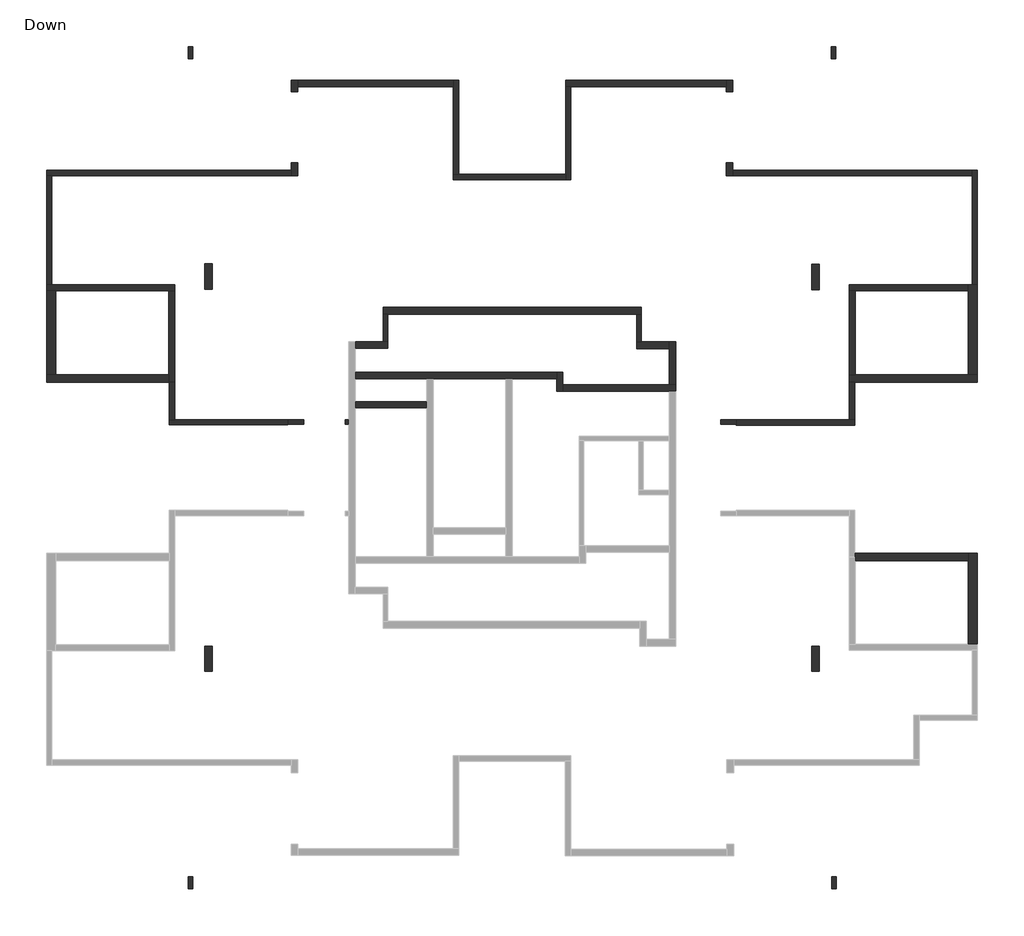
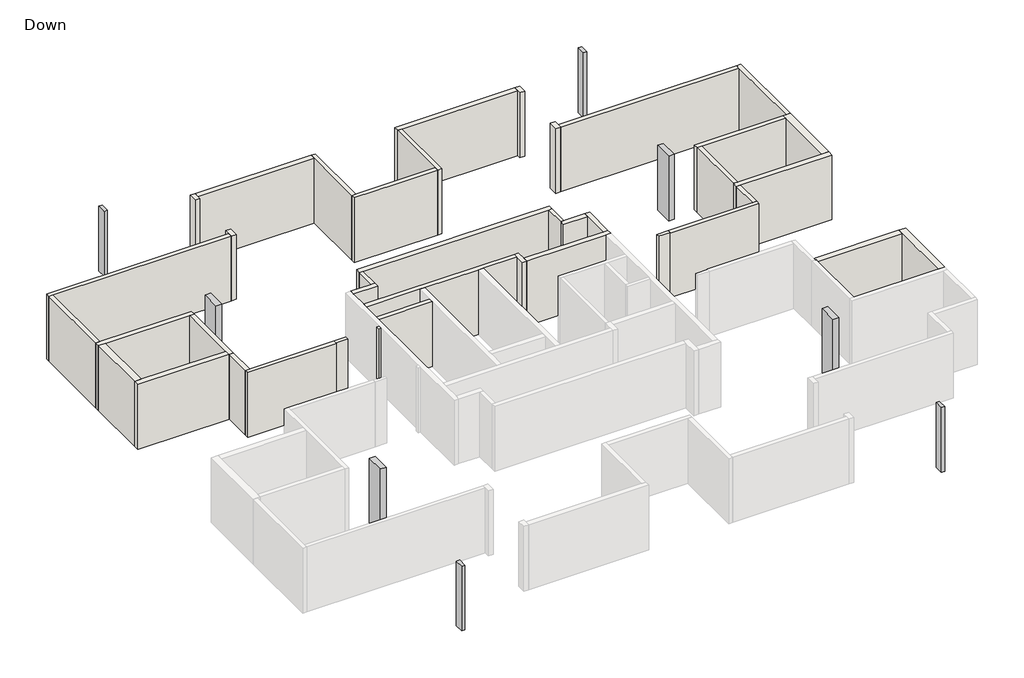
# One storey, part 2 of 2: 40 walls, 8 columns.
"""IFC4 building model written with IfcOpenShell, lengths in millimetres."""

from ifc_helpers import new_model, si_unit, origin, place, context, project, spatial, faceted_brep, element, save

model = new_model("IFC4")

# Units and contexts
model_context = context("Model", 3, world=origin())
ifc_project = project(units=[si_unit("LENGTHUNIT", "METRE", prefix="MILLI")], contexts=[model_context])

# Site, building, storey
site = spatial("IfcSite", under=ifc_project)
building = spatial("IfcBuilding", under=site)
storey = spatial("IfcBuildingStorey", under=building, Name="Down", Elevation=0.0)

# Columns
placement = place(None, origin())
element("IfcColumn", 1, ObjectType="Concrete Rectengular Column : 15/40", at=placement, inside=storey, context=model_context, shape_type="Brep", body=[
    faceted_brep([(7161.4479352, -14720.0113915, 0.0), (7161.4479352, -15120.0113915, 0.0), (7011.4479352, -15120.0113915, 0.0), (7011.4479352, -14720.0113915, 0.0), (7161.4479352, -14720.0113915, 3070.0), (7161.4479352, -15120.0113915, 3070.0), (7161.4479352, -14720.0113915, 2870.0), (7011.4479352, -15120.0113915, 3070.0), (7011.4479352, -15120.0113915, 2870.0), (7011.4479352, -14720.0113915, 3070.0), (7011.4479352, -14720.0113915, 2870.0)], [[[0, 1, 2, 3]], [[4, 5, 1, 0, 6]], [[5, 7, 8, 2, 1]], [[7, 9, 10, 3, 2, 8]], [[9, 4, 6, 0, 3, 10]], [[4, 9, 7, 5]]]),
])
element("IfcColumn", 2, ObjectType="Concrete Rectengular Column : 15/40", at=placement, inside=storey, context=model_context, shape_type="Brep", body=[
    faceted_brep([(-14313.9862657, -14720.0113915, 0.0), (-14313.9862657, -15120.0113915, 0.0), (-14463.9862657, -15120.0113915, 0.0), (-14463.9862657, -14720.0113915, 0.0), (-14313.9862657, -14720.0113915, 3070.0), (-14313.9862657, -15120.0113915, 3070.0), (-14313.9862657, -15120.0113915, 2870.0), (-14313.9862657, -14720.0113915, 2870.0), (-14463.9862657, -15120.0113915, 3070.0), (-14463.9862657, -14720.0113915, 3070.0), (-14463.9862657, -14720.0113915, 2870.0)], [[[0, 1, 2, 3]], [[4, 5, 6, 1, 0, 7]], [[5, 8, 2, 1, 6]], [[8, 9, 10, 3, 2]], [[9, 4, 7, 0, 3, 10]], [[4, 9, 8, 5]]]),
])
element("IfcColumn", 3, ObjectType="Concrete Rectengular Column : 15/40", at=placement, inside=storey, context=model_context, shape_type="Brep", body=[
    faceted_brep([(-14317.8223989, 12998.5060921, 0.0), (-14317.8223989, 12598.5060921, 0.0), (-14467.8223989, 12598.5060921, 0.0), (-14467.8223989, 12998.5060921, 0.0), (-14317.8223989, 12998.5060921, 3070.0), (-14317.8223989, 12598.5060921, 3070.0), (-14317.8223989, 12598.5060921, 2870.0), (-14467.8223989, 12598.5060921, 3070.0), (-14467.8223989, 12598.5060921, 2870.0), (-14467.8223989, 12998.5060921, 3070.0)], [[[0, 1, 2, 3]], [[4, 5, 6, 1, 0]], [[5, 7, 8, 2, 1, 6]], [[7, 9, 3, 2, 8]], [[9, 4, 0, 3]], [[4, 9, 7, 5]]]),
])
element("IfcColumn", 4, ObjectType="Concrete Rectengular Column : 15/40", at=placement, inside=storey, context=model_context, shape_type="Brep", body=[
    faceted_brep([(7142.0982792, 12598.507588, 0.0), (6992.0982792, 12598.507588, 0.0), (6992.0982792, 12998.507588, 0.0), (7142.0982792, 12998.507588, 0.0), (7142.0982792, 12598.507588, 3070.0), (7142.0982792, 12598.507588, 2870.0), (7142.0982792, 12998.507588, 3070.0), (6992.0982792, 12998.507588, 2870.0), (6992.0982792, 12998.507588, 3070.0), (6992.0982792, 12598.507588, 2870.0), (6992.0982792, 12598.507588, 3070.0)], [[[0, 1, 2, 3]], [[4, 5, 0, 3, 6]], [[6, 3, 2, 7, 8]], [[8, 7, 2, 1, 9, 10]], [[10, 9, 1, 0, 5, 4]], [[4, 6, 8, 10]]]),
])
element("IfcColumn", 5, ObjectType="Concrete Rectengular Column : 25/85", at=placement, inside=storey, context=model_context, shape_type="Brep", body=[
    faceted_brep([(-13656.3416868, -7010.4989795, 0.0), (-13656.3416868, -7860.4989795, 0.0), (-13906.3416868, -7860.4989795, 0.0), (-13906.3416868, -7010.4989795, 0.0), (-13656.3416868, -7010.4989795, 3070.0), (-13656.3416868, -7860.4989795, 3070.0), (-13656.3416868, -7860.4989795, 2870.0), (-13656.3416868, -7010.4989795, 2870.0), (-13906.3416868, -7860.4989795, 3070.0), (-13906.3416868, -7860.4989795, 2870.0), (-13906.3416868, -7010.4989795, 3070.0), (-13906.3416868, -7010.4989795, 2870.0)], [[[0, 1, 2, 3]], [[4, 5, 6, 1, 0, 7]], [[5, 8, 9, 2, 1, 6]], [[8, 10, 11, 3, 2, 9]], [[10, 4, 7, 0, 3, 11]], [[4, 10, 8, 5]]]),
])
element("IfcColumn", 6, ObjectType="Concrete Rectengular Column : 25/85", at=placement, inside=storey, context=model_context, shape_type="Brep", body=[
    faceted_brep([(6603.8022343, -7010.4989795, 0.0), (6603.8022343, -7860.4989795, 0.0), (6353.8022343, -7860.4989795, 0.0), (6353.8022343, -7010.4989795, 0.0), (6603.8022343, -7010.4989795, 3070.0), (6603.8022343, -7860.4989795, 3070.0), (6603.8022343, -7860.4989795, 2870.0), (6603.8022343, -7010.4989795, 2870.0), (6353.8022343, -7860.4989795, 3070.0), (6353.8022343, -7860.4989795, 2870.0), (6353.8022343, -7010.4989795, 3070.0), (6353.8022343, -7010.4989795, 2870.0)], [[[0, 1, 2, 3]], [[4, 5, 6, 1, 0, 7]], [[5, 8, 9, 2, 1, 6]], [[8, 10, 11, 3, 2, 9]], [[10, 4, 7, 0, 3, 11]], [[4, 10, 8, 5]]]),
])
element("IfcColumn", 7, ObjectType="Concrete Rectengular Column : 25/85", at=placement, inside=storey, context=model_context, shape_type="Brep", body=[
    faceted_brep([(-13656.3416868, 5740.9327236, 0.0), (-13656.3416868, 4890.9327236, 0.0), (-13906.3416868, 4890.9327236, 0.0), (-13906.3416868, 5740.9327236, 0.0), (-13656.3416868, 5740.9327236, 3070.0), (-13656.3416868, 4890.9327236, 3070.0), (-13656.3416868, 4890.9327236, 2870.0), (-13656.3416868, 5740.9327236, 2870.0), (-13906.3416868, 4890.9327236, 3070.0), (-13906.3416868, 4890.9327236, 2870.0), (-13906.3416868, 5740.9327236, 3070.0), (-13906.3416868, 5740.9327236, 2870.0)], [[[0, 1, 2, 3]], [[4, 5, 6, 1, 0, 7]], [[5, 8, 9, 2, 1, 6]], [[8, 10, 11, 3, 2, 9]], [[10, 4, 7, 0, 3, 11]], [[4, 10, 8, 5]]]),
])
element("IfcColumn", 8, ObjectType="Concrete Rectengular Column : 25/85", at=placement, inside=storey, context=model_context, shape_type="Brep", body=[
    faceted_brep([(6602.4824065, 5738.9914362, 0.0), (6602.4824065, 4888.9914362, 0.0), (6352.4824065, 4888.9914362, 0.0), (6352.4824065, 5738.9914362, 0.0), (6602.4824065, 5738.9914362, 3070.0), (6602.4824065, 4888.9914362, 3070.0), (6602.4824065, 4888.9914362, 2870.0), (6602.4824065, 5738.9914362, 2870.0), (6352.4824065, 4888.9914362, 3070.0), (6352.4824065, 4888.9914362, 2870.0), (6352.4824065, 5738.9914362, 3070.0), (6352.4824065, 5738.9914362, 2870.0)], [[[0, 1, 2, 3]], [[4, 5, 6, 1, 0, 7]], [[5, 8, 9, 2, 1, 6]], [[8, 10, 11, 3, 2, 9]], [[10, 4, 7, 0, 3, 11]], [[4, 10, 8, 5]]]),
])

# Walls
element("IfcWall", 9, ObjectType="15", at=placement, inside=storey, context=model_context, shape_type="Brep", body=[
    faceted_brep([(-10610.0280472, 546.2654793, 0.0), (-11137.3486135, 546.2654793, 0.0), (-11137.3486135, 546.2654793, 2870.0), (-11137.3486135, 546.2654793, 3070.0), (-10610.0280472, 546.2654793, 3070.0), (-10610.0280472, 396.2654793, 0.0), (-10610.0280472, 396.2654793, 2920.0), (-10610.0280472, 396.2654793, 3070.0), (-11137.3486135, 396.2654793, 3070.0), (-11137.3486135, 396.2654793, 2920.0), (-11137.3486135, 396.2654793, 0.0), (-10610.0280472, 396.7654793, 3070.0)], [[[0, 1, 2, 3, 4]], [[5, 6, 7, 8, 9, 10]], [[1, 0, 5, 10]], [[3, 2, 1, 10, 9, 8]], [[4, 3, 8, 7, 11]], [[0, 4, 11, 7, 6, 5]]]),
])
element("IfcWall", 10, ObjectType="15", at=placement, inside=storey, context=model_context, shape_type="Brep", body=[
    faceted_brep([(-9219.5481077, 396.2654793, 0.0), (-9111.0923752, 396.2654793, 0.0), (-9111.0923752, 396.2654793, 2920.0), (-9111.0923752, 396.2654793, 3070.0), (-9219.5481077, 396.2654793, 3070.0), (-9219.5481077, 396.2654793, 2920.0), (-9219.5481077, 546.2654793, 0.0), (-9219.5481077, 546.2654793, 3070.0), (-9111.0923752, 546.2654793, 3070.0), (-9111.0923752, 546.2654793, 2870.0), (-9111.0923752, 546.2654793, 0.0), (-9219.5481077, 396.7654793, 3070.0)], [[[0, 1, 2, 3, 4, 5]], [[6, 7, 8, 9, 10]], [[1, 0, 6, 10]], [[4, 3, 8, 7, 11]], [[0, 5, 4, 11, 7, 6]], [[3, 2, 1, 10, 9, 8]]]),
])
element("IfcWall", 11, ObjectType="15", at=placement, inside=storey, context=model_context, shape_type="Brep", body=[
    faceted_brep([(508.1725561, 4069.1186218, 0.0), (508.1725561, 3137.988413, 0.0), (508.1725561, 3137.988413, 3070.0), (508.1725561, 4069.1186218, 3070.0), (508.1725561, 4069.1186218, 2870.0), (658.1725561, 4069.1186218, 0.0), (658.1725561, 4069.1186218, 3070.0), (658.1725561, 3137.988413, 3070.0), (658.1725561, 3137.988413, 2870.0), (658.1725561, 3137.988413, 0.0)], [[[0, 1, 2, 3, 4]], [[5, 6, 7, 8, 9]], [[1, 0, 5, 9]], [[3, 2, 7, 6]], [[2, 1, 9, 8, 7]], [[0, 4, 3, 6, 5]]]),
])
element("IfcWall", 12, ObjectType="15", at=placement, inside=storey, context=model_context, shape_type="Brep", body=[
    faceted_brep([(-7960.7109614, 4069.1186218, 0.0), (-7960.7109614, 3141.8256682, 0.0), (-7960.7109614, 3141.8256682, 2870.0), (-7960.7109614, 3141.8256682, 3070.0), (-7960.7109614, 4069.1186218, 3070.0), (-7810.7109614, 4069.1186218, 0.0), (-7810.7109614, 4069.1186218, 2870.0), (-7810.7109614, 4069.1186218, 3070.0), (-7810.7109614, 3141.8256682, 3070.0), (-7810.7109614, 3141.8256682, 0.0)], [[[0, 1, 2, 3, 4]], [[5, 6, 7, 8, 9]], [[1, 0, 5, 9]], [[4, 3, 8, 7]], [[3, 2, 1, 9, 8]], [[0, 4, 7, 6, 5]]]),
])
element("IfcWall", 13, ObjectType="15", at=placement, inside=storey, context=model_context, shape_type="Brep", body=[
    faceted_brep([(3307.48852, 390.6860076, 0.0), (3822.84243, 390.6860076, 0.0), (3822.84243, 390.6860076, 2920.0), (3822.84243, 390.6860076, 3070.0), (3307.48852, 390.6860076, 3070.0), (3307.48852, 540.6860076, 0.0), (3307.48852, 540.6860076, 3070.0), (3822.84243, 540.6860076, 3070.0), (3822.84243, 540.6860076, 0.0)], [[[0, 1, 2, 3, 4]], [[5, 6, 7, 8]], [[1, 0, 5, 8]], [[3, 2, 1, 8, 7]], [[4, 3, 7, 6]], [[0, 4, 6, 5]]]),
])
element("IfcWall", 14, ObjectType="18", at=placement, inside=storey, context=model_context, shape_type="Brep", body=[
    faceted_brep([(-11137.3486135, 546.7503763, 0.0), (-14913.3730612, 546.7503763, 0.0), (-15093.3730612, 546.7503763, 0.0), (-15093.3730612, 546.7503763, 3070.0), (-14913.3730612, 546.7503763, 3070.0), (-11137.3486135, 546.7503763, 3070.0), (-11137.3486135, 546.7503763, 2870.0), (-11137.3486135, 366.7503763, 0.0), (-11137.3486135, 366.7503763, 3070.0), (-15093.3730612, 366.7503763, 3070.0), (-15093.3730612, 366.7503763, 0.0), (-11137.3486135, 546.2654793, 0.0), (-11137.3486135, 396.2654793, 0.0), (-11137.3486135, 396.2654793, 3070.0), (-11137.3486135, 546.2654793, 3070.0)], [[[0, 1, 2, 3, 4, 5, 6]], [[7, 8, 9, 10]], [[2, 1, 0, 11, 12, 7, 10]], [[5, 4, 3, 9, 8, 13, 14]], [[0, 6, 5, 14, 13, 8, 7, 12, 11]], [[3, 2, 10, 9]]]),
])
element("IfcWall", 15, ObjectType="18", at=placement, inside=storey, context=model_context, shape_type="Brep", body=[
    faceted_brep([(3822.84243, 360.6860076, 0.0), (7782.84243, 360.6860076, 0.0), (7782.84243, 360.6860076, 3070.0), (3822.84243, 360.6860076, 3070.0), (3822.84243, 540.6860076, 0.0), (3822.84243, 540.6860076, 3070.0), (7602.84243, 540.6860076, 3070.0), (7782.84243, 540.6860076, 3070.0), (7782.84243, 540.6860076, 0.0), (7602.84243, 540.6860076, 0.0), (3822.84243, 390.6860076, 0.0), (3822.84243, 390.6860076, 3070.0)], [[[0, 1, 2, 3]], [[4, 5, 6, 7, 8, 9]], [[1, 0, 10, 4, 9, 8]], [[3, 2, 7, 6, 5, 11]], [[0, 3, 11, 5, 4, 10]], [[2, 1, 8, 7]]]),
])
element("IfcWall", 16, ObjectType="18", at=placement, inside=storey, context=model_context, shape_type="Brep", body=[
    faceted_brep([(7782.84243, 540.6860076, 0.0), (7782.84243, 1793.8824455, 0.0), (7782.84243, 1793.8824455, 3070.0), (7782.84243, 540.6860076, 3070.0), (7602.84243, 540.6860076, 0.0), (7602.84243, 540.6860076, 2870.0), (7602.84243, 540.6860076, 3070.0), (7602.84243, 1793.8824455, 3070.0), (7602.84243, 1793.8824455, 0.0)], [[[0, 1, 2, 3]], [[4, 5, 6, 7, 8]], [[1, 0, 4, 8]], [[3, 2, 7, 6]], [[0, 3, 6, 5, 4]], [[2, 1, 8, 7]]]),
])
element("IfcWall", 17, ObjectType="18", at=placement, inside=storey, context=model_context, shape_type="Brep", body=[
    faceted_brep([(11699.3119283, 8871.9429548, 0.0), (11699.3119283, 8691.9429548, 0.0), (11699.3119283, 5041.1223427, 0.0), (11699.3119283, 5041.1223427, 2870.0), (11699.3119283, 5041.1223427, 3070.0), (11699.3119283, 8691.9429548, 3070.0), (11699.3119283, 8871.9429548, 3070.0), (11879.3119283, 8871.9429548, 0.0), (11879.3119283, 8871.9429548, 3070.0), (11879.3119283, 5041.1223427, 3070.0), (11879.3119283, 5041.1223427, 0.0)], [[[0, 1, 2, 3, 4, 5, 6]], [[7, 8, 9, 10]], [[2, 1, 0, 7, 10]], [[6, 5, 4, 9, 8]], [[0, 6, 8, 7]], [[4, 3, 2, 10, 9]]]),
])
element("IfcWall", 18, ObjectType="18", at=placement, inside=storey, context=model_context, shape_type="Brep", body=[
    faceted_brep([(11699.3119283, 8871.9429548, 0.0), (3719.7179522, 8871.9429548, 0.0), (3719.7179522, 8871.9429548, 2870.0), (3719.7179522, 8871.9429548, 3070.0), (7142.0982792, 8871.9429548, 3070.0), (11699.3119283, 8871.9429548, 3070.0), (11699.3119283, 8691.9429548, 0.0), (11699.3119283, 8691.9429548, 2870.0), (11699.3119283, 8691.9429548, 3070.0), (3719.7179522, 8691.9429548, 3070.0), (3719.7179522, 8691.9429548, 0.0)], [[[0, 1, 2, 3, 4, 5]], [[6, 7, 8, 9, 10]], [[1, 0, 6, 10]], [[5, 4, 3, 9, 8]], [[0, 5, 8, 7, 6]], [[3, 2, 1, 10, 9]]]),
])
element("IfcWall", 19, ObjectType="18", at=placement, inside=storey, context=model_context, shape_type="Brep", body=[
    faceted_brep([(-1870.723263, 11650.5628693, 0.0), (-1870.723263, 8728.0720008, 0.0), (-1870.723263, 8548.0720008, 0.0), (-1870.723263, 8548.0720008, 3070.0), (-1870.723263, 8728.0720008, 3070.0), (-1870.723263, 11650.5628693, 3070.0), (-1690.723263, 11650.5628693, 0.0), (-1690.723263, 11650.5628693, 2870.0), (-1690.723263, 11650.5628693, 3070.0), (-1690.723263, 8548.0720008, 3070.0), (-1690.723263, 8548.0720008, 2870.0), (-1690.723263, 8548.0720008, 0.0)], [[[0, 1, 2, 3, 4, 5]], [[6, 7, 8, 9, 10, 11]], [[2, 1, 0, 6, 11]], [[5, 4, 3, 9, 8]], [[0, 5, 8, 7, 6]], [[3, 2, 11, 10, 9]]]),
])
element("IfcWall", 20, ObjectType="18", at=placement, inside=storey, context=model_context, shape_type="Brep", body=[
    faceted_brep([(-1870.723263, 8728.0720008, 0.0), (-5431.0686661, 8728.0720008, 0.0), (-5611.0686661, 8728.0720008, 0.0), (-5611.3302453, 8728.0720008, 0.0), (-5611.3302453, 8728.0720008, 2870.0), (-5611.3302453, 8728.0720008, 3070.0), (-5611.0686661, 8728.0720008, 3070.0), (-5431.0686661, 8728.0720008, 3070.0), (-1870.723263, 8728.0720008, 3070.0), (-1870.723263, 8548.0720008, 0.0), (-1870.723263, 8548.0720008, 3070.0), (-3553.3678079, 8548.0720008, 3070.0), (-3753.3678079, 8548.0720008, 3070.0), (-5611.3302453, 8548.0720008, 3070.0), (-5611.3302453, 8548.0720008, 2870.0), (-5611.3302453, 8548.0720008, 0.0)], [[[0, 1, 2, 3, 4, 5, 6, 7, 8]], [[9, 10, 11, 12, 13, 14, 15]], [[3, 2, 1, 0, 9, 15]], [[5, 4, 3, 15, 14, 13]], [[8, 7, 6, 5, 13, 12, 11, 10]], [[0, 8, 10, 9]]]),
])
element("IfcWall", 21, ObjectType="18", at=placement, inside=storey, context=model_context, shape_type="Brep", body=[
    faceted_brep([(-5611.0686661, 11870.5628693, 0.0), (-5611.0686661, 11650.5628693, 0.0), (-5611.0686661, 8728.0720008, 0.0), (-5611.0686661, 8728.0720008, 2870.0), (-5611.0686661, 8728.0720008, 3070.0), (-5611.0686661, 11650.5628693, 3070.0), (-5611.0686661, 11870.5628693, 3070.0), (-5431.0686661, 11870.5628693, 0.0), (-5431.0686661, 11870.5628693, 3070.0), (-5431.0686661, 8728.0720008, 3070.0), (-5431.0686661, 8728.0720008, 0.0)], [[[0, 1, 2, 3, 4, 5, 6]], [[7, 8, 9, 10]], [[2, 1, 0, 7, 10]], [[6, 5, 4, 9, 8]], [[4, 3, 2, 10, 9]], [[0, 6, 8, 7]]]),
])
element("IfcWall", 22, ObjectType="18", at=placement, inside=storey, context=model_context, shape_type="Brep", body=[
    faceted_brep([(-11033.4765376, 8871.6813756, 0.0), (-19193.0086039, 8871.6813756, 0.0), (-19193.0086039, 8871.6813756, 3070.0), (-14467.8223989, 8871.6813756, 3070.0), (-11033.4765376, 8871.6813756, 3070.0), (-11033.4765376, 8871.6813756, 2870.0), (-11033.4765376, 8691.6813756, 0.0), (-11033.4765376, 8691.6813756, 3070.0), (-19013.0086039, 8691.6813756, 3070.0), (-19193.0086039, 8691.6813756, 3070.0), (-19193.0086039, 8691.6813756, 0.0), (-19013.0086039, 8691.6813756, 0.0)], [[[0, 1, 2, 3, 4, 5]], [[6, 7, 8, 9, 10, 11]], [[1, 0, 6, 11, 10]], [[4, 3, 2, 9, 8, 7]], [[2, 1, 10, 9]], [[0, 5, 4, 7, 6]]]),
])
element("IfcWall", 23, ObjectType="18", at=placement, inside=storey, context=model_context, shape_type="Brep", body=[
    faceted_brep([(-19193.0086039, 8691.6813756, 0.0), (-19193.0086039, 5045.3187304, 0.0), (-19193.0086039, 5045.3187304, 3070.0), (-19193.0086039, 8691.6813756, 3070.0), (-19013.0086039, 8691.6813756, 0.0), (-19013.0086039, 8691.6813756, 2870.0), (-19013.0086039, 8691.6813756, 3070.0), (-19013.0086039, 5045.3187304, 3070.0), (-19013.0086039, 5045.3187304, 2870.0), (-19013.0086039, 5045.3187304, 0.0)], [[[0, 1, 2, 3]], [[4, 5, 6, 7, 8, 9]], [[1, 0, 4, 9]], [[3, 2, 7, 6]], [[0, 3, 6, 5, 4]], [[2, 1, 9, 8, 7]]]),
])
element("IfcWall", 24, ObjectType="18", at=placement, inside=storey, context=model_context, shape_type="Brep", body=[
    faceted_brep([(-15093.3730612, 1793.8819255, 0.0), (-15093.3730612, 546.7503763, 0.0), (-15093.3730612, 546.7503763, 3070.0), (-15093.3730612, 1793.8819255, 3070.0), (-14913.3730612, 1793.8819255, 0.0), (-14913.3730612, 1793.8819255, 2870.0), (-14913.3730612, 1793.8819255, 3070.0), (-14913.3730612, 546.7503763, 3070.0), (-14913.3730612, 546.7503763, 2870.0), (-14913.3730612, 546.7503763, 0.0)], [[[0, 1, 2, 3]], [[4, 5, 6, 7, 8, 9]], [[1, 0, 4, 9]], [[3, 2, 7, 6]], [[0, 3, 6, 5, 4]], [[2, 1, 9, 8, 7]]]),
])
element("IfcWall", 25, ObjectType="20", at=placement, inside=storey, context=model_context, shape_type="Brep", body=[
    faceted_brep([(-2155.2421674, 2134.3048342, 0.0), (-2155.2421674, 1914.3048342, 0.0), (-2155.2421674, 1493.9448789, 0.0), (-2155.2421674, 1493.9448789, 2870.0), (-2155.2421674, 1493.9448789, 3070.0), (-2155.2421674, 1914.3048342, 3070.0), (-2155.2421674, 2134.3048342, 3070.0), (-1955.2421674, 2134.3048342, 0.0), (-1955.2421674, 2134.3048342, 2870.0), (-1955.2421674, 2134.3048342, 3070.0), (-1955.2421674, 1713.9448789, 3070.0), (-1955.2421674, 1493.9448789, 3070.0), (-1955.2421674, 1493.9448789, 0.0), (-1955.2421674, 1713.9448789, 0.0)], [[[0, 1, 2, 3, 4, 5, 6]], [[7, 8, 9, 10, 11, 12, 13]], [[2, 1, 0, 7, 13, 12]], [[6, 5, 4, 11, 10, 9]], [[4, 3, 2, 12, 11]], [[0, 6, 9, 8, 7]]]),
])
element("IfcWall", 26, ObjectType="20", at=placement, inside=storey, context=model_context, shape_type="Brep", body=[
    faceted_brep([(11579.3119283, 5041.1223427, 0.0), (7602.84243, 5041.1223427, 0.0), (7602.84243, 5041.1223427, 2870.0), (7602.84243, 5041.1223427, 3070.0), (11579.3119283, 5041.1223427, 3070.0), (11579.3119283, 4841.1223427, 0.0), (11579.3119283, 4841.1223427, 2870.0), (11579.3119283, 4841.1223427, 3070.0), (7802.84243, 4841.1223427, 3070.0), (7602.84243, 4841.1223427, 3070.0), (7602.84243, 4841.1223427, 0.0), (7802.84243, 4841.1223427, 0.0)], [[[0, 1, 2, 3, 4]], [[5, 6, 7, 8, 9, 10, 11]], [[1, 0, 5, 11, 10]], [[4, 3, 9, 8, 7]], [[3, 2, 1, 10, 9]], [[0, 4, 7, 6, 5]]]),
])
element("IfcWall", 27, ObjectType="20", at=placement, inside=storey, context=model_context, shape_type="Brep", body=[
    faceted_brep([(7802.84243, 2043.8824455, 0.0), (7802.84243, 4841.1223427, 0.0), (7802.84243, 4841.1223427, 2870.0), (7802.84243, 4841.1223427, 3070.0), (7802.84243, 2043.8824455, 3070.0), (7802.84243, 2043.8824455, 2870.0), (7602.84243, 2043.8824455, 0.0), (7602.84243, 2043.8824455, 3070.0), (7602.84243, 4841.1223427, 3070.0), (7602.84243, 4841.1223427, 0.0)], [[[0, 1, 2, 3, 4, 5]], [[6, 7, 8, 9]], [[1, 0, 6, 9]], [[4, 3, 8, 7]], [[3, 2, 1, 9, 8]], [[0, 5, 4, 7, 6]]]),
])
element("IfcWall", 28, ObjectType="20", at=placement, inside=storey, context=model_context, shape_type="Brep", body=[
    faceted_brep([(-19193.0086039, 4845.3187304, 0.0), (-18893.0086039, 4845.3187304, 0.0), (-15113.1120804, 4845.3187304, 0.0), (-14913.1120804, 4845.3187304, 0.0), (-14913.1120804, 4845.3187304, 3070.0), (-15113.1120804, 4845.3187304, 3070.0), (-18893.0086039, 4845.3187304, 3070.0), (-19193.0086039, 4845.3187304, 3070.0), (-19193.0086039, 5045.3187304, 0.0), (-19193.0086039, 5045.3187304, 3070.0), (-19013.0086039, 5045.3187304, 3070.0), (-14913.1120804, 5045.3187304, 3070.0), (-14913.1120804, 5045.3187304, 2870.0), (-14913.1120804, 5045.3187304, 0.0), (-19013.0086039, 5045.3187304, 0.0)], [[[0, 1, 2, 3, 4, 5, 6, 7]], [[8, 9, 10, 11, 12, 13, 14]], [[3, 2, 1, 0, 8, 14, 13]], [[7, 6, 5, 4, 11, 10, 9]], [[0, 7, 9, 8]], [[4, 3, 13, 12, 11]]]),
])
element("IfcWall", 29, ObjectType="20", at=placement, inside=storey, context=model_context, shape_type="Brep", body=[
    faceted_brep([(-15113.1120804, 4845.3187304, 0.0), (-15113.1120804, 2043.8819255, 0.0), (-15113.1120804, 1793.8819255, 0.0), (-15113.1120804, 1793.8819255, 3070.0), (-15113.1120804, 2043.8819255, 3070.0), (-15113.1120804, 4845.3187304, 3070.0), (-15113.1120804, 4845.3187304, 2870.0), (-14913.1120804, 4845.3187304, 0.0), (-14913.1120804, 4845.3187304, 3070.0), (-14913.1120804, 1793.8819255, 3070.0), (-14913.1120804, 1793.8819255, 2870.0), (-14913.1120804, 1793.8819255, 0.0), (-14913.3730612, 1793.8819255, 0.0), (-15093.3730612, 1793.8819255, 0.0), (-15093.3730612, 1793.8819255, 3070.0), (-14913.3730612, 1793.8819255, 3070.0)], [[[0, 1, 2, 3, 4, 5, 6]], [[7, 8, 9, 10, 11]], [[2, 1, 0, 7, 11, 12, 13]], [[5, 4, 3, 14, 15, 9, 8]], [[0, 6, 5, 8, 7]], [[3, 2, 13, 12, 11, 10, 9, 15, 14]]]),
])
element("IfcWall", 30, ObjectType="20", at=placement, inside=storey, context=model_context, shape_type="Brep", body=[
    faceted_brep([(-8891.0923752, 942.6898033, 0.0), (-6498.4263718, 942.6898033, 0.0), (-6498.4263718, 942.6898033, 2870.0), (-6498.4263718, 942.6898033, 3070.0), (-8891.0923752, 942.6898033, 3070.0), (-8891.0923752, 942.6898033, 2870.0), (-8891.0923752, 1142.6898033, 0.0), (-8891.0923752, 1142.6898033, 3070.0), (-6498.4263718, 1142.6898033, 3070.0), (-6498.4263718, 1142.6898033, 0.0)], [[[0, 1, 2, 3, 4, 5]], [[6, 7, 8, 9]], [[1, 0, 6, 9]], [[4, 3, 8, 7]], [[0, 5, 4, 7, 6]], [[3, 2, 1, 9, 8]]]),
])
element("IfcWall", 31, ObjectType="22", at=placement, inside=storey, context=model_context, shape_type="Brep", body=[
    faceted_brep([(-8891.0923752, 2921.8256682, 0.0), (-7810.7109614, 2921.8256682, 0.0), (-7810.7109614, 2921.8256682, 2870.0), (-7810.7109614, 2921.8256682, 3070.0), (-8891.0923752, 2921.8256682, 3070.0), (-8891.0923752, 2921.8256682, 2870.0), (-8891.0923752, 3141.8256682, 0.0), (-8891.0923752, 3141.8256682, 3070.0), (-7960.7109614, 3141.8256682, 3070.0), (-7810.7109614, 3141.8256682, 3070.0), (-7810.7109614, 3141.8256682, 0.0), (-7960.7109614, 3141.8256682, 0.0)], [[[0, 1, 2, 3, 4, 5]], [[6, 7, 8, 9, 10, 11]], [[1, 0, 6, 11, 10]], [[4, 3, 9, 8, 7]], [[0, 5, 4, 7, 6]], [[3, 2, 1, 10, 9]]]),
])
element("IfcWall", 32, ObjectType="22", at=placement, inside=storey, context=model_context, shape_type="Brep", body=[
    faceted_brep([(-7960.7109614, 4069.1186218, 0.0), (-7810.7109614, 4069.1186218, 0.0), (508.1725561, 4069.1186218, 0.0), (658.1725561, 4069.1186218, 0.0), (658.1725561, 4069.1186218, 3070.0), (508.1725561, 4069.1186218, 3070.0), (-7810.7109614, 4069.1186218, 3070.0), (-7960.7109614, 4069.1186218, 3070.0), (-7960.7109614, 4289.1186218, 0.0), (-7960.7109614, 4289.1186218, 2870.0), (-7960.7109614, 4289.1186218, 3070.0), (-3753.3678079, 4289.1186218, 3070.0), (-3553.3678079, 4289.1186218, 3070.0), (658.1725561, 4289.1186218, 3070.0), (658.1725561, 4289.1186218, 2870.0), (658.1725561, 4289.1186218, 0.0)], [[[0, 1, 2, 3, 4, 5, 6, 7]], [[8, 9, 10, 11, 12, 13, 14, 15]], [[3, 2, 1, 0, 8, 15]], [[7, 6, 5, 4, 13, 12, 11, 10]], [[0, 7, 10, 9, 8]], [[4, 3, 15, 14, 13]]]),
])
element("IfcWall", 33, ObjectType="22", at=placement, inside=storey, context=model_context, shape_type="Brep", body=[
    faceted_brep([(-8891.0923752, 1914.3048342, 0.0), (-6498.4263718, 1914.3048342, 0.0), (-6278.4263718, 1914.3048342, 0.0), (-3873.0437953, 1914.3048342, 0.0), (-3653.0437953, 1914.3048342, 0.0), (-2155.2421674, 1914.3048342, 0.0), (-2155.2421674, 1914.3048342, 2870.0), (-2155.2421674, 1914.3048342, 3070.0), (-3653.0437953, 1914.3048342, 3070.0), (-3873.0437953, 1914.3048342, 3070.0), (-6278.4263718, 1914.3048342, 3070.0), (-6498.4263718, 1914.3048342, 3070.0), (-8891.0923752, 1914.3048342, 3070.0), (-8891.0923752, 2134.3048342, 0.0), (-8891.0923752, 2134.3048342, 2870.0), (-8891.0923752, 2134.3048342, 3070.0), (-2155.2421674, 2134.3048342, 3070.0), (-2155.2421674, 2134.3048342, 0.0)], [[[0, 1, 2, 3, 4, 5, 6, 7, 8, 9, 10, 11, 12]], [[13, 14, 15, 16, 17]], [[5, 4, 3, 2, 1, 0, 13, 17]], [[12, 11, 10, 9, 8, 7, 16, 15]], [[7, 6, 5, 17, 16]], [[0, 12, 15, 14, 13]]]),
])
element("IfcWall", 34, ObjectType="22", at=placement, inside=storey, context=model_context, shape_type="Brep", body=[
    faceted_brep([(-1955.2421674, 1493.9448789, 0.0), (1589.3005209, 1493.9448789, 0.0), (1809.3005209, 1493.9448789, 0.0), (1809.3005209, 1493.9448789, 3070.0), (1589.3005209, 1493.9448789, 3070.0), (-1955.2421674, 1493.9448789, 3070.0), (-1955.2421674, 1713.9448789, 0.0), (-1955.2421674, 1713.9448789, 2870.0), (-1955.2421674, 1713.9448789, 3070.0), (1589.3005209, 1713.9448789, 3070.0), (1809.3005209, 1713.9448789, 3070.0), (1809.3005209, 1713.9448789, 0.0), (1589.3005209, 1713.9448789, 0.0)], [[[0, 1, 2, 3, 4, 5]], [[6, 7, 8, 9, 10, 11, 12]], [[2, 1, 0, 6, 12, 11]], [[5, 4, 3, 10, 9, 8]], [[3, 2, 11, 10]], [[0, 5, 8, 7, 6]]]),
])
element("IfcWall", 35, ObjectType="22", at=placement, inside=storey, context=model_context, shape_type="Brep", body=[
    faceted_brep([(1589.3005209, 3137.988413, 0.0), (1589.3005209, 2917.988413, 0.0), (1589.3005209, 1713.9448789, 0.0), (1589.3005209, 1713.9448789, 2870.0), (1589.3005209, 1713.9448789, 3070.0), (1589.3005209, 2917.988413, 3070.0), (1589.3005209, 3137.988413, 3070.0), (1809.3005209, 3137.988413, 0.0), (1809.3005209, 3137.988413, 2870.0), (1809.3005209, 3137.988413, 3070.0), (1809.3005209, 1713.9448789, 3070.0), (1809.3005209, 1713.9448789, 0.0)], [[[0, 1, 2, 3, 4, 5, 6]], [[7, 8, 9, 10, 11]], [[2, 1, 0, 7, 11]], [[6, 5, 4, 10, 9]], [[0, 6, 9, 8, 7]], [[4, 3, 2, 11, 10]]]),
])
element("IfcWall", 36, ObjectType="22", at=placement, inside=storey, context=model_context, shape_type="Brep", body=[
    faceted_brep([(1589.3005209, 3137.988413, 0.0), (658.1725561, 3137.988413, 0.0), (508.1725561, 3137.988413, 0.0), (508.1725561, 3137.988413, 3070.0), (658.1725561, 3137.988413, 3070.0), (1589.3005209, 3137.988413, 3070.0), (1589.3005209, 2917.988413, 0.0), (1589.3005209, 2917.988413, 2870.0), (1589.3005209, 2917.988413, 3070.0), (508.1725561, 2917.988413, 3070.0), (508.1725561, 2917.988413, 2870.0), (508.1725561, 2917.988413, 0.0)], [[[0, 1, 2, 3, 4, 5]], [[6, 7, 8, 9, 10, 11]], [[2, 1, 0, 6, 11]], [[5, 4, 3, 9, 8]], [[0, 5, 8, 7, 6]], [[3, 2, 11, 10, 9]]]),
])
element("IfcWall", 37, ObjectType="22", at=placement, inside=storey, context=model_context, shape_type="Brep", body=[
    faceted_brep([(3499.7179522, 11870.5628693, 0.0), (-1870.723263, 11870.5628693, 0.0), (-1870.723263, 11870.5628693, 3070.0), (3499.7179522, 11870.5628693, 3070.0), (3499.7179522, 11650.5628693, 0.0), (3499.7179522, 11650.5628693, 2870.0), (3499.7179522, 11650.5628693, 3070.0), (-1690.723263, 11650.5628693, 3070.0), (-1870.723263, 11650.5628693, 3070.0), (-1870.723263, 11650.5628693, 0.0), (-1690.723263, 11650.5628693, 0.0)], [[[0, 1, 2, 3]], [[4, 5, 6, 7, 8, 9, 10]], [[1, 0, 4, 10, 9]], [[3, 2, 8, 7, 6]], [[2, 1, 9, 8]], [[0, 3, 6, 5, 4]]]),
])
element("IfcWall", 38, ObjectType="22", at=placement, inside=storey, context=model_context, shape_type="Brep", body=[
    faceted_brep([(-5611.0686661, 11870.5628693, 0.0), (-10813.4765376, 11870.5628693, 0.0), (-10813.4765376, 11870.5628693, 3070.0), (-5611.0686661, 11870.5628693, 3070.0), (-5611.0686661, 11650.5628693, 0.0), (-5611.0686661, 11650.5628693, 2870.0), (-5611.0686661, 11650.5628693, 3070.0), (-10813.4765376, 11650.5628693, 3070.0), (-10813.4765376, 11650.5628693, 2870.0), (-10813.4765376, 11650.5628693, 0.0)], [[[0, 1, 2, 3]], [[4, 5, 6, 7, 8, 9]], [[1, 0, 4, 9]], [[3, 2, 7, 6]], [[0, 3, 6, 5, 4]], [[2, 1, 9, 8, 7]]]),
])
element("IfcWall", 39, ObjectType="22", at=placement, inside=storey, context=model_context, shape_type="Brep", body=[
    faceted_brep([(3499.7179522, 11870.5628693, 0.0), (3499.7179522, 11650.5628693, 0.0), (3499.7179522, 11490.5628693, 0.0), (3499.7179522, 11490.5628693, 2920.0), (3499.7179522, 11490.5628693, 3070.0), (3499.7179522, 11650.5628693, 3070.0), (3499.7179522, 11870.5628693, 3070.0), (3499.7179522, 11870.5628693, 2870.0), (3719.7179522, 11870.5628693, 0.0), (3719.7179522, 11870.5628693, 2870.0), (3719.7179522, 11870.5628693, 3070.0), (3719.7179522, 11490.5628693, 3070.0), (3719.7179522, 11490.5628693, 2920.0), (3719.7179522, 11490.5628693, 0.0)], [[[0, 1, 2, 3, 4, 5, 6, 7]], [[8, 9, 10, 11, 12, 13]], [[2, 1, 0, 8, 13]], [[4, 3, 2, 13, 12, 11]], [[6, 5, 4, 11, 10]], [[0, 7, 6, 10, 9, 8]]]),
])
element("IfcWall", 40, ObjectType="22", at=placement, inside=storey, context=model_context, shape_type="Brep", body=[
    faceted_brep([(3719.7179522, 8691.9429548, 0.0), (3719.7179522, 8871.9429548, 0.0), (3719.7179522, 9111.9429548, 0.0), (3719.7179522, 9111.9429548, 2920.0), (3719.7179522, 9111.9429548, 3070.0), (3719.7179522, 8871.9429548, 3070.0), (3719.7179522, 8691.9429548, 3070.0), (3499.7179522, 8691.9429548, 0.0), (3499.7179522, 8691.9429548, 2870.0), (3499.7179522, 8691.9429548, 3070.0), (3499.7179522, 9111.9429548, 3070.0), (3499.7179522, 9111.9429548, 2920.0), (3499.7179522, 9111.9429548, 0.0)], [[[0, 1, 2, 3, 4, 5, 6]], [[7, 8, 9, 10, 11, 12]], [[2, 1, 0, 7, 12]], [[4, 3, 2, 12, 11, 10]], [[6, 5, 4, 10, 9]], [[0, 6, 9, 8, 7]]]),
])
element("IfcWall", 41, ObjectType="22", at=placement, inside=storey, context=model_context, shape_type="Brep", body=[
    faceted_brep([(-11033.4765376, 11870.5628693, 0.0), (-11033.4765376, 11490.5628693, 0.0), (-11033.4765376, 11490.5628693, 2920.0), (-11033.4765376, 11490.5628693, 3070.0), (-11033.4765376, 11870.5628693, 3070.0), (-11033.4765376, 11870.5628693, 2870.0), (-10813.4765376, 11870.5628693, 0.0), (-10813.4765376, 11870.5628693, 2870.0), (-10813.4765376, 11870.5628693, 3070.0), (-10813.4765376, 11650.5628693, 3070.0), (-10813.4765376, 11490.5628693, 3070.0), (-10813.4765376, 11490.5628693, 2920.0), (-10813.4765376, 11490.5628693, 0.0), (-10813.4765376, 11650.5628693, 0.0)], [[[0, 1, 2, 3, 4, 5]], [[6, 7, 8, 9, 10, 11, 12, 13]], [[1, 0, 6, 13, 12]], [[3, 2, 1, 12, 11, 10]], [[4, 3, 10, 9, 8]], [[0, 5, 4, 8, 7, 6]]]),
])
element("IfcWall", 42, ObjectType="22", at=placement, inside=storey, context=model_context, shape_type="Brep", body=[
    faceted_brep([(-10813.4765376, 8691.6813756, 0.0), (-10813.4765376, 9111.6813756, 0.0), (-10813.4765376, 9111.6813756, 2920.0), (-10813.4765376, 9111.6813756, 3070.0), (-10813.4765376, 8691.6813756, 3070.0), (-10813.4765376, 8691.6813756, 2870.0), (-11033.4765376, 8691.6813756, 0.0), (-11033.4765376, 8691.6813756, 3070.0), (-11033.4765376, 8871.6813756, 3070.0), (-11033.4765376, 9111.6813756, 3070.0), (-11033.4765376, 9111.6813756, 2920.0), (-11033.4765376, 9111.6813756, 0.0), (-11033.4765376, 8871.6813756, 0.0)], [[[0, 1, 2, 3, 4, 5]], [[6, 7, 8, 9, 10, 11, 12]], [[1, 0, 6, 12, 11]], [[3, 2, 1, 11, 10, 9]], [[4, 3, 9, 8, 7]], [[0, 5, 4, 7, 6]]]),
])
element("IfcWall", 43, ObjectType="25", at=placement, inside=storey, context=model_context, shape_type="Brep", body=[
    faceted_brep([(11579.3119283, -3916.1341463, 0.0), (7780.4432059, -3916.1341463, 0.0), (7780.4432059, -3916.1341463, 3070.0), (11579.3119283, -3916.1341463, 3070.0), (11579.3119283, -4166.1341463, 0.0), (11579.3119283, -4166.1341463, 2870.0), (11579.3119283, -4166.1341463, 3070.0), (7800.4432059, -4166.1341463, 3070.0), (7800.4432059, -4166.1341463, 2870.0), (7800.4432059, -4166.1341463, 0.0), (7800.4432059, -4041.1341463, 0.0), (7780.4432059, -4041.1341463, 0.0), (7780.4432059, -4041.1341463, 3070.0), (7800.4432059, -4041.1341463, 3070.0)], [[[0, 1, 2, 3]], [[4, 5, 6, 7, 8, 9]], [[1, 0, 4, 9, 10, 11]], [[3, 2, 12, 13, 7, 6]], [[0, 3, 6, 5, 4]], [[2, 1, 11, 12]], [[11, 10, 13, 12]], [[10, 9, 8, 7, 13]]]),
])
element("IfcWall", 44, ObjectType="25", at=placement, inside=storey, context=model_context, shape_type="Brep", body=[
    faceted_brep([(11879.3119283, 2043.8824455, 0.0), (11579.3119283, 2043.8824455, 0.0), (7802.84243, 2043.8824455, 0.0), (7602.84243, 2043.8824455, 0.0), (7602.84243, 2043.8824455, 3070.0), (7802.84243, 2043.8824455, 3070.0), (11579.3119283, 2043.8824455, 3070.0), (11879.3119283, 2043.8824455, 3070.0), (11879.3119283, 1793.8824455, 0.0), (11879.3119283, 1793.8824455, 3070.0), (7782.84243, 1793.8824455, 3070.0), (7602.84243, 1793.8824455, 3070.0), (7602.84243, 1793.8824455, 0.0), (7782.84243, 1793.8824455, 0.0)], [[[0, 1, 2, 3, 4, 5, 6, 7]], [[8, 9, 10, 11, 12, 13]], [[3, 2, 1, 0, 8, 13, 12]], [[7, 6, 5, 4, 11, 10, 9]], [[4, 3, 12, 11]], [[0, 7, 9, 8]]]),
])
element("IfcWall", 45, ObjectType="25", at=placement, inside=storey, context=model_context, shape_type="Brep", body=[
    faceted_brep([(-15113.1120804, 2043.8819255, 0.0), (-18893.0086039, 2043.8819255, 0.0), (-19193.0086039, 2043.8819255, 0.0), (-19193.0086039, 2043.8819255, 3070.0), (-18893.0086039, 2043.8819255, 3070.0), (-15113.1120804, 2043.8819255, 3070.0), (-15113.1120804, 2043.8819255, 2870.0), (-15113.1120804, 1793.8819255, 0.0), (-15113.1120804, 1793.8819255, 3070.0), (-19193.0086039, 1793.8819255, 3070.0), (-19193.0086039, 1793.8819255, 0.0)], [[[0, 1, 2, 3, 4, 5, 6]], [[7, 8, 9, 10]], [[2, 1, 0, 7, 10]], [[5, 4, 3, 9, 8]], [[0, 6, 5, 8, 7]], [[3, 2, 10, 9]]]),
])
element("IfcWall", 46, ObjectType="30", at=placement, inside=storey, context=model_context, shape_type="Brep", body=[
    faceted_brep([(11879.3119283, -6953.7627402, 0.0), (11879.3119283, -3916.1341463, 0.0), (11879.3119283, -3916.1341463, 3070.0), (11879.3119283, -6953.7627402, 3070.0), (11579.3119283, -6953.7627402, 0.0), (11579.3119283, -6953.7627402, 2870.0), (11579.3119283, -6953.7627402, 3070.0), (11579.3119283, -4166.1341463, 3070.0), (11579.3119283, -3916.1341463, 3070.0), (11579.3119283, -3916.1341463, 0.0), (11579.3119283, -4166.1341463, 0.0)], [[[0, 1, 2, 3]], [[4, 5, 6, 7, 8, 9, 10]], [[1, 0, 4, 10, 9]], [[3, 2, 8, 7, 6]], [[0, 3, 6, 5, 4]], [[2, 1, 9, 8]]]),
])
element("IfcWall", 47, ObjectType="30", at=placement, inside=storey, context=model_context, shape_type="Brep", body=[
    faceted_brep([(11879.3119283, 2043.8824455, 0.0), (11879.3119283, 5041.1223427, 0.0), (11879.3119283, 5041.1223427, 3070.0), (11879.3119283, 2043.8824455, 3070.0), (11579.3119283, 2043.8824455, 0.0), (11579.3119283, 2043.8824455, 2870.0), (11579.3119283, 2043.8824455, 3070.0), (11579.3119283, 4841.1223427, 3070.0), (11579.3119283, 5041.1223427, 3070.0), (11579.3119283, 5041.1223427, 0.0), (11579.3119283, 4841.1223427, 0.0), (11699.3119283, 5041.1223427, 0.0), (11699.3119283, 5041.1223427, 3070.0)], [[[0, 1, 2, 3]], [[4, 5, 6, 7, 8, 9, 10]], [[1, 0, 4, 10, 9, 11]], [[3, 2, 12, 8, 7, 6]], [[0, 3, 6, 5, 4]], [[2, 1, 11, 9, 8, 12]]]),
])
element("IfcWall", 48, ObjectType="30", at=placement, inside=storey, context=model_context, shape_type="Brep", body=[
    faceted_brep([(-18893.0086039, 2043.8819255, 0.0), (-18893.0086039, 4845.3187304, 0.0), (-18893.0086039, 4845.3187304, 2870.0), (-18893.0086039, 4845.3187304, 3070.0), (-18893.0086039, 2043.8819255, 3070.0), (-18893.0086039, 2043.8819255, 2870.0), (-19193.0086039, 2043.8819255, 0.0), (-19193.0086039, 2043.8819255, 3070.0), (-19193.0086039, 4845.3187304, 3070.0), (-19193.0086039, 4845.3187304, 0.0)], [[[0, 1, 2, 3, 4, 5]], [[6, 7, 8, 9]], [[1, 0, 6, 9]], [[4, 3, 8, 7]], [[0, 5, 4, 7, 6]], [[3, 2, 1, 9, 8]]]),
])

save(model, "model.ifc")

# Revit data of these elements
# Type "Concrete Rectengular Column : 15/40"
#   b = 15 cm
#   h = 40 cm
#   Structural Material [instance default] = Concrete, Cast-in-Place - B30
# Type "Concrete Rectengular Column : 25/85"
#   b = 25 cm
#   h = 85 cm
#   Structural Material [instance default] = Concrete, Cast-in-Place - B30
# Type "15"
#   Layers, outside or top first: 15 cm "Concrete" (function 1)
# Type "18"
#   Layers, outside or top first: 18 cm "Concrete" (function 1)
# Type "20"
#   Layers, outside or top first: 20 cm "Concrete" (function 1)
# Type "22"
#   Layers, outside or top first: 22 cm "Concrete" (function 1)
# Type "25"
#   Layers, outside or top first: 25 cm "Concrete" (function 1)
# Type "30"
#   Layers, outside or top first: 30 cm "Concrete" (function 1)
# Element 1 (IfcColumn, "Concrete Rectengular Column : 15/40")
#   Comments = ""
#   Mark = "C1"
#   SOFiSTiK_AMG_Comments = ""
#   SOFiSTiK_AMG_Scheduled = yes
#   SOFiSTiK_AMG_Adjusted = yes
#   Structural Material = Concrete
#   Phase Created = New Construction
#   Materials on its faces: "Concrete"
# Element 2 (IfcColumn, "Concrete Rectengular Column : 15/40")
#   Comments = ""
#   Mark = "C2"
#   SOFiSTiK_AMG_Comments = ""
#   SOFiSTiK_AMG_Scheduled = yes
#   SOFiSTiK_AMG_Adjusted = yes
#   Structural Material = Concrete
#   Phase Created = New Construction
#   Materials on its faces: "Concrete"
# Element 3 (IfcColumn, "Concrete Rectengular Column : 15/40")
#   Comments = ""
#   Mark = "C3"
#   SOFiSTiK_AMG_Comments = ""
#   SOFiSTiK_AMG_Scheduled = yes
#   SOFiSTiK_AMG_Adjusted = yes
#   Structural Material = Concrete
#   Phase Created = New Construction
#   Materials on its faces: "Concrete"
# Element 4 (IfcColumn, "Concrete Rectengular Column : 15/40")
#   Comments = ""
#   Mark = "C4"
#   SOFiSTiK_AMG_Comments = ""
#   SOFiSTiK_AMG_Scheduled = yes
#   SOFiSTiK_AMG_Adjusted = yes
#   Structural Material = Concrete
#   Phase Created = New Construction
#   Materials on its faces: "Concrete"
# Element 5 (IfcColumn, "Concrete Rectengular Column : 25/85")
#   Comments = ""
#   Mark = "C5"
#   SOFiSTiK_AMG_Comments = ""
#   SOFiSTiK_AMG_Scheduled = yes
#   SOFiSTiK_AMG_Adjusted = yes
#   Structural Material = Concrete
#   Phase Created = New Construction
#   Materials on its faces: "Concrete"
# Element 6 (IfcColumn, "Concrete Rectengular Column : 25/85")
#   Comments = ""
#   Mark = "C6"
#   SOFiSTiK_AMG_Comments = ""
#   SOFiSTiK_AMG_Scheduled = yes
#   SOFiSTiK_AMG_Adjusted = yes
#   Structural Material = Concrete
#   Phase Created = New Construction
#   Materials on its faces: "Concrete"
# Element 7 (IfcColumn, "Concrete Rectengular Column : 25/85")
#   Comments = ""
#   Mark = "C7"
#   SOFiSTiK_AMG_Comments = ""
#   SOFiSTiK_AMG_Scheduled = yes
#   SOFiSTiK_AMG_Adjusted = yes
#   Structural Material = Concrete
#   Phase Created = New Construction
#   Materials on its faces: "Concrete"
# Element 8 (IfcColumn, "Concrete Rectengular Column : 25/85")
#   Comments = ""
#   Mark = "C8"
#   SOFiSTiK_AMG_Comments = ""
#   SOFiSTiK_AMG_Scheduled = yes
#   SOFiSTiK_AMG_Adjusted = yes
#   Structural Material = Concrete
#   Phase Created = New Construction
#   Materials on its faces: "Concrete"
# Element 9 (IfcWall, "15")
#   Comments = ""
#   Mark = "W74"
#   SOFiSTiK_EdgeZones = "W74"
#   SOFiSTiK_AMG_Comments = ""
#   Top Offset = 0 cm
#   Base Offset = 0 cm
#   wall height = 307 cm
#   SOFiSTiK_AMG_Scheduled = yes
#   SOFiSTiK_AMG_Adjusted = yes
#   Phase Created = New Construction
#   Base Constraint = Down
#   Top Constraint = Typical Floor
#   Materials on its faces: "Concrete"
# Element 10 (IfcWall, "15")
#   Comments = ""
#   Mark = "W75"
#   SOFiSTiK_EdgeZones = "W75"
#   SOFiSTiK_AMG_Comments = "Too Short /"
#   Top Offset = 0 cm
#   Base Offset = 0 cm
#   wall height = 307 cm
#   SOFiSTiK_AMG_Scheduled = yes
#   SOFiSTiK_AMG_Adjusted = yes
#   Phase Created = New Construction
#   Base Constraint = Down
#   Top Constraint = Typical Floor
#   Materials on its faces: "Concrete"
# Element 11 (IfcWall, "15")
#   Comments = ""
#   Mark = "W76"
#   SOFiSTiK_EdgeZones = "W76"
#   SOFiSTiK_AMG_Comments = ""
#   Top Offset = 0 cm
#   Base Offset = 0 cm
#   wall height = 307 cm
#   SOFiSTiK_AMG_Scheduled = yes
#   SOFiSTiK_AMG_Adjusted = yes
#   Phase Created = New Construction
#   Base Constraint = Down
#   Top Constraint = Typical Floor
#   Materials on its faces: "Concrete"
# Element 12 (IfcWall, "15")
#   Comments = ""
#   Mark = "W77"
#   SOFiSTiK_EdgeZones = "W77"
#   SOFiSTiK_AMG_Comments = ""
#   Top Offset = 0 cm
#   Base Offset = 0 cm
#   wall height = 307 cm
#   SOFiSTiK_AMG_Scheduled = yes
#   SOFiSTiK_AMG_Adjusted = yes
#   Phase Created = New Construction
#   Base Constraint = Down
#   Top Constraint = Typical Floor
#   Materials on its faces: "Concrete"
# Element 13 (IfcWall, "15")
#   Comments = ""
#   Mark = "W78"
#   SOFiSTiK_EdgeZones = "W78"
#   SOFiSTiK_AMG_Comments = ""
#   Top Offset = 0 cm
#   Base Offset = 0 cm
#   wall height = 307 cm
#   SOFiSTiK_AMG_Scheduled = yes
#   SOFiSTiK_AMG_Adjusted = yes
#   Phase Created = New Construction
#   Base Constraint = Down
#   Top Constraint = Typical Floor
#   Materials on its faces: "Concrete"
# Element 14 (IfcWall, "18")
#   Comments = ""
#   Mark = "W18"
#   SOFiSTiK_EdgeZones = "W18"
#   SOFiSTiK_AMG_Comments = ""
#   Top Offset = 0 cm
#   Base Offset = 0 cm
#   wall height = 307 cm
#   SOFiSTiK_AMG_Scheduled = yes
#   SOFiSTiK_AMG_Adjusted = yes
#   Phase Created = New Construction
#   Base Constraint = Down
#   Top Constraint = Typical Floor
#   Materials on its faces: "Concrete"
# Element 15 (IfcWall, "18")
#   Comments = ""
#   Mark = "W19"
#   SOFiSTiK_EdgeZones = "W19"
#   SOFiSTiK_AMG_Comments = ""
#   Top Offset = 0 cm
#   Base Offset = 0 cm
#   wall height = 307 cm
#   SOFiSTiK_AMG_Scheduled = yes
#   SOFiSTiK_AMG_Adjusted = yes
#   Phase Created = New Construction
#   Base Constraint = Down
#   Top Constraint = Typical Floor
#   Materials on its faces: "Concrete"
# Element 16 (IfcWall, "18")
#   Comments = ""
#   Mark = "W20"
#   SOFiSTiK_EdgeZones = "W20"
#   SOFiSTiK_AMG_Comments = ""
#   Top Offset = 0 cm
#   Base Offset = 0 cm
#   wall height = 307 cm
#   SOFiSTiK_AMG_Scheduled = yes
#   SOFiSTiK_AMG_Adjusted = yes
#   Phase Created = New Construction
#   Base Constraint = Down
#   Top Constraint = Typical Floor
#   Materials on its faces: "Concrete"
# Element 17 (IfcWall, "18")
#   Comments = ""
#   Mark = "W21"
#   SOFiSTiK_EdgeZones = "W21"
#   SOFiSTiK_AMG_Comments = ""
#   Top Offset = 0 cm
#   Base Offset = 0 cm
#   wall height = 307 cm
#   SOFiSTiK_AMG_Scheduled = yes
#   SOFiSTiK_AMG_Adjusted = yes
#   Phase Created = New Construction
#   Base Constraint = Down
#   Top Constraint = Typical Floor
#   Materials on its faces: "Concrete"
# Element 18 (IfcWall, "18")
#   Comments = ""
#   Mark = "W22"
#   SOFiSTiK_EdgeZones = "W22"
#   SOFiSTiK_AMG_Comments = ""
#   Top Offset = 0 cm
#   Base Offset = 0 cm
#   wall height = 307 cm
#   SOFiSTiK_AMG_Scheduled = yes
#   SOFiSTiK_AMG_Adjusted = yes
#   Phase Created = New Construction
#   Base Constraint = Down
#   Top Constraint = Typical Floor
#   Materials on its faces: "Concrete"
# Element 19 (IfcWall, "18")
#   Comments = ""
#   Mark = "W23"
#   SOFiSTiK_EdgeZones = "W23"
#   SOFiSTiK_AMG_Comments = ""
#   Top Offset = 0 cm
#   Base Offset = 0 cm
#   wall height = 307 cm
#   SOFiSTiK_AMG_Scheduled = yes
#   SOFiSTiK_AMG_Adjusted = yes
#   Phase Created = New Construction
#   Base Constraint = Down
#   Top Constraint = Typical Floor
#   Materials on its faces: "Concrete"
# Element 20 (IfcWall, "18")
#   Comments = ""
#   Mark = "W24"
#   SOFiSTiK_EdgeZones = "W24"
#   SOFiSTiK_AMG_Comments = ""
#   Top Offset = 0 cm
#   Base Offset = 0 cm
#   wall height = 307 cm
#   SOFiSTiK_AMG_Scheduled = yes
#   SOFiSTiK_AMG_Adjusted = yes
#   Phase Created = New Construction
#   Base Constraint = Down
#   Top Constraint = Typical Floor
#   Materials on its faces: "Concrete"
# Element 21 (IfcWall, "18")
#   Comments = ""
#   Mark = "W25"
#   SOFiSTiK_EdgeZones = "W25"
#   SOFiSTiK_AMG_Comments = ""
#   Top Offset = 0 cm
#   Base Offset = 0 cm
#   wall height = 307 cm
#   SOFiSTiK_AMG_Scheduled = yes
#   SOFiSTiK_AMG_Adjusted = yes
#   Phase Created = New Construction
#   Base Constraint = Down
#   Top Constraint = Typical Floor
#   Materials on its faces: "Concrete"
# Element 22 (IfcWall, "18")
#   Comments = ""
#   Mark = "W26"
#   SOFiSTiK_EdgeZones = "W26"
#   SOFiSTiK_AMG_Comments = ""
#   Top Offset = 0 cm
#   Base Offset = 0 cm
#   wall height = 307 cm
#   SOFiSTiK_AMG_Scheduled = yes
#   SOFiSTiK_AMG_Adjusted = yes
#   Phase Created = New Construction
#   Base Constraint = Down
#   Top Constraint = Typical Floor
#   Materials on its faces: "Concrete"
# Element 23 (IfcWall, "18")
#   Comments = ""
#   Mark = "W27"
#   SOFiSTiK_EdgeZones = "W27"
#   SOFiSTiK_AMG_Comments = ""
#   Top Offset = 0 cm
#   Base Offset = 0 cm
#   wall height = 307 cm
#   SOFiSTiK_AMG_Scheduled = yes
#   SOFiSTiK_AMG_Adjusted = yes
#   Phase Created = New Construction
#   Base Constraint = Down
#   Top Constraint = Typical Floor
#   Materials on its faces: "Concrete"
# Element 24 (IfcWall, "18")
#   Comments = ""
#   Mark = "W28"
#   SOFiSTiK_EdgeZones = "W28"
#   SOFiSTiK_AMG_Comments = ""
#   Top Offset = 0 cm
#   Base Offset = 0 cm
#   wall height = 307 cm
#   SOFiSTiK_AMG_Scheduled = yes
#   SOFiSTiK_AMG_Adjusted = yes
#   Phase Created = New Construction
#   Base Constraint = Down
#   Top Constraint = Typical Floor
#   Materials on its faces: "Concrete"
# Element 25 (IfcWall, "20")
#   Comments = ""
#   Mark = "W36"
#   SOFiSTiK_EdgeZones = "W36"
#   SOFiSTiK_AMG_Comments = ""
#   Top Offset = 0 cm
#   Base Offset = 0 cm
#   wall height = 307 cm
#   SOFiSTiK_AMG_Scheduled = yes
#   SOFiSTiK_AMG_Adjusted = yes
#   Phase Created = New Construction
#   Base Constraint = Down
#   Top Constraint = Typical Floor
#   Materials on its faces: "Concrete"
# Element 26 (IfcWall, "20")
#   Comments = ""
#   Mark = "W37"
#   SOFiSTiK_EdgeZones = "W37"
#   SOFiSTiK_AMG_Comments = ""
#   Top Offset = 0 cm
#   Base Offset = 0 cm
#   wall height = 307 cm
#   SOFiSTiK_AMG_Scheduled = yes
#   SOFiSTiK_AMG_Adjusted = yes
#   Phase Created = New Construction
#   Base Constraint = Down
#   Top Constraint = Typical Floor
#   Materials on its faces: "Concrete"
# Element 27 (IfcWall, "20")
#   Comments = ""
#   Mark = "W38"
#   SOFiSTiK_EdgeZones = "W38"
#   SOFiSTiK_AMG_Comments = ""
#   Top Offset = 0 cm
#   Base Offset = 0 cm
#   wall height = 307 cm
#   SOFiSTiK_AMG_Scheduled = yes
#   SOFiSTiK_AMG_Adjusted = yes
#   Phase Created = New Construction
#   Base Constraint = Down
#   Top Constraint = Typical Floor
#   Materials on its faces: "Concrete"
# Element 28 (IfcWall, "20")
#   Comments = ""
#   Mark = "W39"
#   SOFiSTiK_EdgeZones = "W39"
#   SOFiSTiK_AMG_Comments = ""
#   Top Offset = 0 cm
#   Base Offset = 0 cm
#   wall height = 307 cm
#   SOFiSTiK_AMG_Scheduled = yes
#   SOFiSTiK_AMG_Adjusted = yes
#   Phase Created = New Construction
#   Base Constraint = Down
#   Top Constraint = Typical Floor
#   Materials on its faces: "Concrete"
# Element 29 (IfcWall, "20")
#   Comments = ""
#   Mark = "W40"
#   SOFiSTiK_EdgeZones = "W40"
#   SOFiSTiK_AMG_Comments = ""
#   Top Offset = 0 cm
#   Base Offset = 0 cm
#   wall height = 307 cm
#   SOFiSTiK_AMG_Scheduled = yes
#   SOFiSTiK_AMG_Adjusted = yes
#   Phase Created = New Construction
#   Base Constraint = Down
#   Top Constraint = Typical Floor
#   Materials on its faces: "Concrete"
# Element 30 (IfcWall, "20")
#   Comments = ""
#   Mark = "W41"
#   SOFiSTiK_EdgeZones = "W41"
#   SOFiSTiK_AMG_Comments = ""
#   Top Offset = 0 cm
#   Base Offset = 0 cm
#   wall height = 307 cm
#   SOFiSTiK_AMG_Scheduled = yes
#   SOFiSTiK_AMG_Adjusted = yes
#   Phase Created = New Construction
#   Base Constraint = Down
#   Top Constraint = Typical Floor
#   Materials on its faces: "Concrete"
# Element 31 (IfcWall, "22")
#   Comments = ""
#   Mark = "W45"
#   SOFiSTiK_EdgeZones = "W45"
#   SOFiSTiK_AMG_Comments = ""
#   Top Offset = 0 cm
#   Base Offset = 0 cm
#   wall height = 307 cm
#   SOFiSTiK_AMG_Scheduled = yes
#   SOFiSTiK_AMG_Adjusted = yes
#   Phase Created = New Construction
#   Base Constraint = Down
#   Top Constraint = Typical Floor
#   Materials on its faces: "Concrete"
# Element 32 (IfcWall, "22")
#   Comments = ""
#   Mark = "W46"
#   SOFiSTiK_EdgeZones = "W46"
#   SOFiSTiK_AMG_Comments = ""
#   Top Offset = 0 cm
#   Base Offset = 0 cm
#   wall height = 307 cm
#   SOFiSTiK_AMG_Scheduled = yes
#   SOFiSTiK_AMG_Adjusted = yes
#   Phase Created = New Construction
#   Base Constraint = Down
#   Top Constraint = Typical Floor
#   Materials on its faces: "Concrete"
# Element 33 (IfcWall, "22")
#   Comments = ""
#   Mark = "W47"
#   SOFiSTiK_EdgeZones = "W47"
#   SOFiSTiK_AMG_Comments = ""
#   Top Offset = 0 cm
#   Base Offset = 0 cm
#   wall height = 307 cm
#   SOFiSTiK_AMG_Scheduled = yes
#   SOFiSTiK_AMG_Adjusted = yes
#   Phase Created = New Construction
#   Base Constraint = Down
#   Top Constraint = Typical Floor
#   Materials on its faces: "Concrete"
# Element 34 (IfcWall, "22")
#   Comments = ""
#   Mark = "W48"
#   SOFiSTiK_EdgeZones = "W48"
#   SOFiSTiK_AMG_Comments = ""
#   Top Offset = 0 cm
#   Base Offset = 0 cm
#   wall height = 307 cm
#   SOFiSTiK_AMG_Scheduled = yes
#   SOFiSTiK_AMG_Adjusted = yes
#   Phase Created = New Construction
#   Base Constraint = Down
#   Top Constraint = Typical Floor
#   Materials on its faces: "Concrete"
# Element 35 (IfcWall, "22")
#   Comments = ""
#   Mark = "W49"
#   SOFiSTiK_EdgeZones = "W49"
#   SOFiSTiK_AMG_Comments = ""
#   Top Offset = 0 cm
#   Base Offset = 0 cm
#   wall height = 307 cm
#   SOFiSTiK_AMG_Scheduled = yes
#   SOFiSTiK_AMG_Adjusted = yes
#   Phase Created = New Construction
#   Base Constraint = Down
#   Top Constraint = Typical Floor
#   Materials on its faces: "Concrete"
# Element 36 (IfcWall, "22")
#   Comments = ""
#   Mark = "W50"
#   SOFiSTiK_EdgeZones = "W50"
